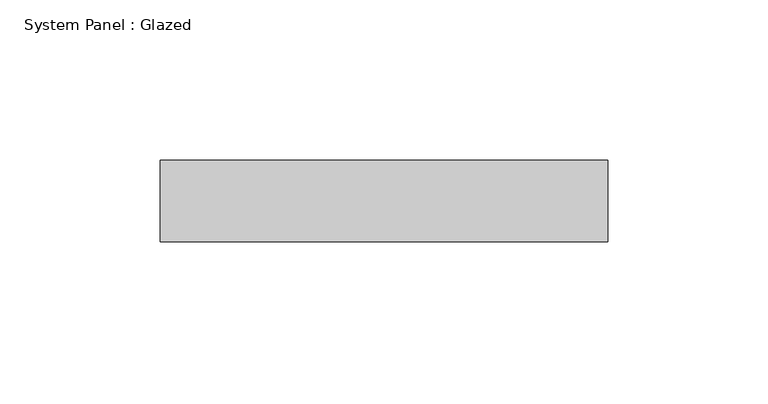
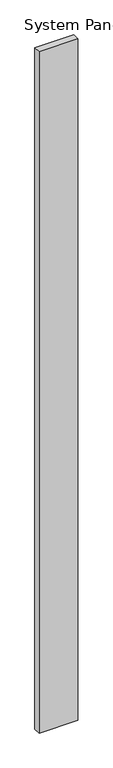
"""IFC4 building model written with IfcOpenShell, lengths in millimetres: plate geometry, System Panel : Glazed."""

import ifcopenshell
import ifcopenshell.guid

model = None  # the IFC model being written
_history = None  # IfcOwnerHistory: only IFC2X3 demands one
_inside = {}  # id of a spatial element -> (the spatial element, [elements in it])
_under = {}  # id of a project, library or spatial element -> (it, [spatial elements below it])
_declared = {}  # id of a project -> (the project, [libraries it declares])
_typed = {}  # id of a type object -> (the type object, [elements of that type])
_made_of = {}  # id of a material, layer set ... -> (it, [elements and type objects made of it])


def new_model(schema):
    """Start an empty IFC model of exactly this schema.

    Asked for "IFC4X3", IfcOpenShell would pick the latest addendum, in which some entities
    have other attributes; the version numbers below select the first issue.
    IFC2X3 requires an IfcOwnerHistory on every rooted entity: one is made here for all.
    """
    global model, _history
    if schema == "IFC4X3":
        model = ifcopenshell.file(schema_version=(4, 3, 0, 0))
    else:
        model = ifcopenshell.file(schema=schema)
    _inside.clear()
    _under.clear()
    _declared.clear()
    _typed.clear()
    _made_of.clear()
    _history = None
    if model.schema == "IFC2X3":
        org = make("IfcOrganization", Name="unknown")
        user = make(
            "IfcPersonAndOrganization",
            ThePerson=make("IfcPerson", FamilyName="unknown"),
            TheOrganization=org,
        )
        app = make(
            "IfcApplication",
            ApplicationDeveloper=org,
            Version="unknown",
            ApplicationFullName="unknown",
            ApplicationIdentifier="unknown",
        )
        _history = make(
            "IfcOwnerHistory",
            OwningUser=user,
            OwningApplication=app,
            ChangeAction="ADDED",
            CreationDate=0,
        )
    return model


def make(cls, **values):
    """One entity of the class cls with the attributes given. An attribute that is None is left unset."""
    return model.create_entity(
        cls, **{name: value for name, value in values.items() if value is not None}
    )


def rooted(cls, **values):
    """An entity with a GlobalId (a new one), such as an element, a storey or a relation."""
    return make(cls, GlobalId=ifcopenshell.guid.new(), OwnerHistory=_history, **values)


def si_unit(unit_type, name, prefix=None):
    """IfcSIUnit, for example si_unit("LENGTHUNIT", "METRE", prefix="MILLI")."""
    return make("IfcSIUnit", UnitType=unit_type, Prefix=prefix, Name=name)


def assignment(units):
    """IfcUnitAssignment: the units of a project."""
    return None if units is None else make("IfcUnitAssignment", Units=units)


def point(xyz):
    """IfcCartesianPoint."""
    return None if xyz is None else make("IfcCartesianPoint", Coordinates=xyz)


def direction(xyz):
    """IfcDirection."""
    return None if xyz is None else make("IfcDirection", DirectionRatios=xyz)


def frame(location, z_axis=None, x_axis=None):
    """IfcAxis2Placement3D, a coordinate frame: its origin and axes. An axis left out is left unset."""
    return make(
        "IfcAxis2Placement3D",
        Location=point(location),
        Axis=direction(z_axis),
        RefDirection=direction(x_axis),
    )


def origin():
    """The frame at (0, 0, 0) with its axes left unset."""
    return frame((0.0, 0.0, 0.0))


def origin_with_axes():
    """The frame at (0, 0, 0) with the z axis (0, 0, 1) and the x axis (1, 0, 0) written out."""
    return frame((0.0, 0.0, 0.0), z_axis=(0.0, 0.0, 1.0), x_axis=(1.0, 0.0, 0.0))


def place(relative_to, where):
    """IfcLocalPlacement: puts the frame where relative to a parent placement (None: the world)."""
    return make(
        "IfcLocalPlacement", PlacementRelTo=relative_to, RelativePlacement=where
    )


def context(
    kind, dimensions, precision=None, world=None, true_north=None, identifier=None
):
    """IfcGeometricRepresentationContext, for example the 3D "Model" context."""
    return make(
        "IfcGeometricRepresentationContext",
        ContextIdentifier=identifier,
        ContextType=kind,
        CoordinateSpaceDimension=dimensions,
        Precision=precision,
        WorldCoordinateSystem=world,
        TrueNorth=true_north,
    )


def project(units=None, contexts=None):
    """IfcProject with its units and contexts."""
    return rooted(
        "IfcProject",
        Name="project",
        RepresentationContexts=contexts,
        UnitsInContext=assignment(units),
    )


def spatial(cls, under=None, at=None, **own):
    """A site, building, storey or space (cls), placed at a placement, below another one or the project."""
    s = rooted(cls, ObjectPlacement=at, **own)
    if under is not None:
        _under.setdefault(under.id(), (under, []))[1].append(s)
    return s


def polyline(points):
    """IfcPolyline through the points."""
    return make("IfcPolyline", Points=[point(p) for p in points])


def outline(outer, holes=None, kind="AREA"):
    """IfcArbitraryClosedProfileDef: a profile drawn as a closed curve; with holes, ...WithVoids."""
    if holes is None:
        return make("IfcArbitraryClosedProfileDef", ProfileType=kind, OuterCurve=outer)
    return make(
        "IfcArbitraryProfileDefWithVoids",
        ProfileType=kind,
        OuterCurve=outer,
        InnerCurves=holes,
    )


def extrude(swept, where, along, depth):
    """IfcExtrudedAreaSolid: the profile swept, set in the frame where, extruded along a direction by depth."""
    return make(
        "IfcExtrudedAreaSolid",
        SweptArea=swept,
        Position=where,
        ExtrudedDirection=direction(along),
        Depth=depth,
    )


def shape(context_of_items, identifier, shape_type, items):
    """IfcShapeRepresentation: the items that make up one representation, for example the "Body"."""
    return make(
        "IfcShapeRepresentation",
        ContextOfItems=context_of_items,
        RepresentationIdentifier=identifier,
        RepresentationType=shape_type,
        Items=items,
    )


def source(mapping_origin, context_of_items, identifier, shape_type, items):
    """IfcRepresentationMap: a shape defined once, which mapped items show again and again."""
    return make(
        "IfcRepresentationMap",
        MappingOrigin=mapping_origin,
        MappedRepresentation=shape(context_of_items, identifier, shape_type, items),
    )


def transform(
    local_origin,
    x_axis=None,
    y_axis=None,
    z_axis=None,
    scale=None,
    scale2=None,
    scale3=None,
    uniform=True,
):
    """IfcCartesianTransformationOperator3D, or its non-uniform kind. x_axis, y_axis, z_axis: its Axis1, 2, 3."""
    if uniform:
        return make(
            "IfcCartesianTransformationOperator3D",
            Axis1=direction(x_axis),
            Axis2=direction(y_axis),
            LocalOrigin=point(local_origin),
            Scale=scale,
            Axis3=direction(z_axis),
        )
    return make(
        "IfcCartesianTransformationOperator3DnonUniform",
        Axis1=direction(x_axis),
        Axis2=direction(y_axis),
        LocalOrigin=point(local_origin),
        Scale=scale,
        Axis3=direction(z_axis),
        Scale2=scale2,
        Scale3=scale3,
    )


def mapped(mapping_source, mapping_target):
    """IfcMappedItem: shows the shape of a source again, moved by a transform."""
    return make(
        "IfcMappedItem", MappingSource=mapping_source, MappingTarget=mapping_target
    )


def made_of(thing, what):
    """Note that an element or type object is made of a material, layer set ...; save() writes the relation."""
    if what is not None:
        _made_of.setdefault(what.id(), (what, []))[1].append(thing)
    return thing


def element(
    cls,
    number,
    at=None,
    inside=None,
    cuts=None,
    type_object=None,
    material=None,
    context=None,
    identifier="Body",
    shape_type=None,
    held_by="IfcProductDefinitionShape",
    body=None,
    shapes=None,
    **own,
):
    """One element of the class cls, such as IfcWall. Its Tag is "e" and its number.

    at: its placement. inside: the storey or other place that contains it. cuts: it is an
    opening in that element (IfcRelVoidsElement). A single representation is given by context,
    identifier, shape_type and body (its items); several are given by shapes. held_by: the class
    of the entity that holds the representations. save() writes the other relations.
    """
    e = rooted(cls, Tag="e%d" % number, ObjectPlacement=at, **own)
    if body is not None:
        shapes = [shape(context, identifier, shape_type, body)]
    if shapes is not None:
        e.Representation = make(held_by, Representations=shapes)
    if inside is not None:
        _inside.setdefault(inside.id(), (inside, []))[1].append(e)
    if cuts is not None:
        rooted(
            "IfcRelVoidsElement", RelatingBuildingElement=cuts, RelatedOpeningElement=e
        )
    if type_object is not None:
        _typed.setdefault(type_object.id(), (type_object, []))[1].append(e)
    return made_of(e, material)


def aggregate(whole, parts):
    """IfcRelAggregates: a whole, such as a stair, and the parts it consists of."""
    return rooted("IfcRelAggregates", RelatingObject=whole, RelatedObjects=parts)


def save(model, path):
    """Write the relations noted so far, then the file.

    IfcRelAggregates (storeys below a building ...), IfcRelContainedInSpatialStructure (elements
    in a storey), IfcRelDefinesByType, IfcRelAssociatesMaterial and IfcRelDeclares: one each for
    every whole, place, type object, material and project.
    """
    for whole, parts in _under.values():
        aggregate(whole, parts)
    for where, things in _inside.values():
        rooted(
            "IfcRelContainedInSpatialStructure",
            RelatedElements=things,
            RelatingStructure=where,
        )
    for kind, things in _typed.values():
        rooted("IfcRelDefinesByType", RelatedObjects=things, RelatingType=kind)
    for what, things in _made_of.values():
        rooted("IfcRelAssociatesMaterial", RelatedObjects=things, RelatingMaterial=what)
    for by, libraries in _declared.values():
        rooted("IfcRelDeclares", RelatingContext=by, RelatedDefinitions=libraries)
    model.write(path)


def system_panel_glazed_a3432af0(model_context):
    return source(origin(), model_context, "Body", "SweptSolid", [
        extrude(outline(polyline([(69.649919, 19.05), (-69.649919, 19.05), (-69.649919, 44.45), (69.649919, 44.45), (69.649919, 19.05)])), origin_with_axes(), (0.0, 0.0, 1.0), 2578.1),
    ])


if __name__ == "__main__":
    model = new_model("IFC4")
    model_context = context("Model", 3, world=origin())
    ifc_project = project(units=[si_unit("LENGTHUNIT", "METRE", prefix="MILLI")], contexts=[model_context])
    site = spatial("IfcSite", under=ifc_project)
    building = spatial("IfcBuilding", under=site)
    placement = place(None, origin())
    system_panel_glazed_shape = system_panel_glazed_a3432af0(model_context)
    element("IfcPlate", 1, ObjectType="System Panel : Glazed", at=placement, inside=building, context=model_context, shape_type="MappedRepresentation", body=[
        mapped(system_panel_glazed_shape, transform((0.0, 0.0, 0.0), x_axis=(1.0, 0.0, 0.0), y_axis=(0.0, 1.0, 0.0), z_axis=(0.0, 0.0, 1.0))),
    ])
    save(model, "model.ifc")

# Revit data of these elements
# Type "System Panel : Glazed"
#   Construction Type Id = "GSP4R"
#   Analytic Construction = "1/8 in Pilkington single glazing"
#   Visual Light Transmittance = 0.9
#   Solar Heat Gain Coefficient = 0.86
#   Heat Transfer Coefficient (U) = 1.18115 BTU/(h·ft²·°F)
#   Define Thermal Properties by = 1
# Element 1 (IfcPlate, "System Panel : Glazed")
#   Materials on its faces: "Glass"
# Materials
#   "Glass": class "Glass", colour RGB 0 128 192, transparency 0.75, Description = "Soda Lime Glass", Cost = 0
